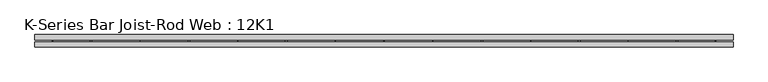
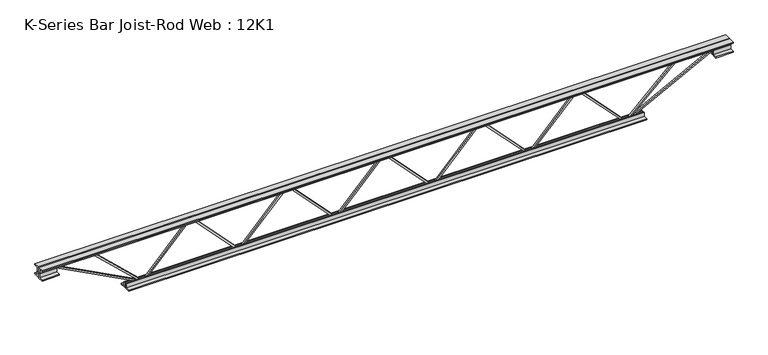
"""IFC4 building model written with IfcOpenShell, lengths in millimetres: beam geometry, K-Series Bar Joist-Rod Web : 12K1."""

from ifc_helpers import new_model, si_unit, frame, origin, place, context, project, spatial, polyline, outline, extrude, source, transform, mapped, element, save


def k_series_bar_joist_rod_web_12k1_58f41b11(model_context):
    return source(origin(), model_context, "Body", "SweptSolid", [
        extrude(outline(polyline([(-141.2875, 283.68625), (-150.8125, 283.68625), (-150.8125, 288.9066515), (141.2875, 566.2429015), (141.2875, 568.5020985), (-150.8125, 845.8383485), (-150.8125, 851.05875), (-141.2875, 851.05875), (-141.2875, 849.9291515), (150.8125, 572.5929015), (150.8125, 562.1520985), (-141.2875, 284.8158485), (-141.2875, 283.68625)])), frame((0.0, -4.7625, 0.0), z_axis=(0.0, 1.0, 0.0), x_axis=(0.0, 0.0, 1.0)), (0.0, 0.0, 1.0), 9.525),
        extrude(outline(polyline([(-141.2875, -283.68625), (-150.8125, -283.68625), (-150.8125, -278.4658485), (141.2875, -1.1295985), (141.2875, 1.1295985), (-150.8125, 278.4658485), (-150.8125, 283.68625), (-141.2875, 283.68625), (-141.2875, 282.5566515), (150.8125, 5.2204015), (150.8125, -5.2204015), (-141.2875, -282.5566515), (-141.2875, -283.68625)])), frame((0.0, -4.7625, 0.0), z_axis=(0.0, 1.0, 0.0), x_axis=(0.0, 0.0, 1.0)), (0.0, 0.0, 1.0), 9.525),
        extrude(outline(polyline([(-141.2875, -851.05875), (-150.8125, -851.05875), (-150.8125, -845.8383485), (141.2875, -568.5020985), (141.2875, -566.2429015), (-150.8125, -288.9066515), (-150.8125, -283.68625), (-141.2875, -283.68625), (-141.2875, -284.8158485), (150.8125, -562.1520985), (150.8125, -572.5929015), (-141.2875, -849.9291515), (-141.2875, -851.05875)])), frame((0.0, -4.7625, 0.0), z_axis=(0.0, 1.0, 0.0), x_axis=(0.0, 0.0, 1.0)), (0.0, 0.0, 1.0), 9.525),
        extrude(outline(polyline([(-141.2875, 851.05875), (-150.8125, 851.05875), (-150.8125, 856.2791515), (141.2875, 1133.6154015), (141.2875, 1135.8745985), (-150.8125, 1413.2108485), (-150.8125, 1418.43125), (-141.2875, 1418.43125), (-141.2875, 1417.3016515), (150.8125, 1139.9654015), (150.8125, 1129.5245985), (-141.2875, 852.1883485), (-141.2875, 851.05875)])), frame((0.0, -4.7625, 0.0), z_axis=(0.0, 1.0, 0.0), x_axis=(0.0, 0.0, 1.0)), (0.0, 0.0, 1.0), 9.525),
        extrude(outline(polyline([(-141.2875, -1418.43125), (-150.8125, -1418.43125), (-150.8125, -1413.2108485), (141.2875, -1135.8745985), (141.2875, -1133.6154015), (-150.8125, -856.2791515), (-150.8125, -851.05875), (-141.2875, -851.05875), (-141.2875, -852.1883485), (150.8125, -1129.5245985), (150.8125, -1139.9654015), (-141.2875, -1417.3016515), (-141.2875, -1418.43125)])), frame((0.0, -4.7625, 0.0), z_axis=(0.0, 1.0, 0.0), x_axis=(0.0, 0.0, 1.0)), (0.0, 0.0, 1.0), 9.525),
        extrude(outline(polyline([(4.7625, 152.4), (36.5125, 152.4), (36.5125, 146.05), (11.1125, 146.05), (11.1125, 120.65), (4.7625, 120.65), (4.7625, 152.4)])), frame((-2028.03125, 0.0, 0.0), z_axis=(1.0, 0.0, 0.0), x_axis=(0.0, 1.0, 0.0)), (0.0, 0.0, 1.0), 4056.0625),
        extrude(outline(polyline([(-4.7625, 152.4), (-4.7625, 120.65), (-11.1125, 120.65), (-11.1125, 146.05), (-36.5125, 146.05), (-36.5125, 152.4), (-4.7625, 152.4)])), frame((-2028.03125, 0.0, 0.0), z_axis=(1.0, 0.0, 0.0), x_axis=(0.0, 1.0, 0.0)), (0.0, 0.0, 1.0), 4056.0625),
        extrude(outline(polyline([(-4.7625, 88.9), (-36.5125, 88.9), (-36.5125, 95.25), (-11.1125, 95.25), (-11.1125, 120.65), (-4.7625, 120.65), (-4.7625, 88.9)])), frame((-2028.03125, 0.0, 0.0), z_axis=(1.0, 0.0, 0.0), x_axis=(0.0, 1.0, 0.0)), (0.0, 0.0, 1.0), 101.6),
        extrude(outline(polyline([(36.5125, 88.9), (4.7625, 88.9), (4.7625, 120.65), (11.1125, 120.65), (11.1125, 95.25), (36.5125, 95.25), (36.5125, 88.9)])), frame((-2028.03125, 0.0, 0.0), z_axis=(1.0, 0.0, 0.0), x_axis=(0.0, 1.0, 0.0)), (0.0, 0.0, 1.0), 101.6),
        extrude(outline(polyline([(4.7625, 88.9), (4.7625, 120.65), (11.1125, 120.65), (11.1125, 95.25), (36.5125, 95.25), (36.5125, 88.9), (4.7625, 88.9)])), frame((1926.43125, 0.0, 0.0), z_axis=(1.0, 0.0, 0.0), x_axis=(0.0, 1.0, 0.0)), (0.0, 0.0, 1.0), 101.6),
        extrude(outline(polyline([(-4.7625, 88.9), (-36.5125, 88.9), (-36.5125, 95.25), (-11.1125, 95.25), (-11.1125, 120.65), (-4.7625, 120.65), (-4.7625, 88.9)])), frame((1926.43125, 0.0, 0.0), z_axis=(1.0, 0.0, 0.0), x_axis=(0.0, 1.0, 0.0)), (0.0, 0.0, 1.0), 101.6),
        extrude(outline(polyline([(4.7625, -152.4), (4.7625, -120.65), (11.1125, -120.65), (11.1125, -146.05), (36.5125, -146.05), (36.5125, -152.4), (4.7625, -152.4)])), frame((-1520.03125, 0.0, 0.0), z_axis=(1.0, 0.0, 0.0), x_axis=(0.0, 1.0, 0.0)), (0.0, 0.0, 1.0), 3040.0625),
        extrude(outline(polyline([(-4.7625, -152.4), (-36.5125, -152.4), (-36.5125, -146.05), (-11.1125, -146.05), (-11.1125, -120.65), (-4.7625, -120.65), (-4.7625, -152.4)])), frame((-1520.03125, 0.0, 0.0), z_axis=(1.0, 0.0, 0.0), x_axis=(0.0, 1.0, 0.0)), (0.0, 0.0, 1.0), 3040.0625),
        extrude(outline(polyline([(0.0, -9.525), (0.0, 0.0), (573.7533355, 0.0), (573.7533355, -9.525), (0.0, -9.525)])), frame((-1928.6450214, 4.7625, 116.4332925), z_axis=(0.4648338989895146, 0.0, 0.8853979028381566), x_axis=(0.8853979028381566, 0.0, -0.4648338989895146)), (0.0, 0.0, 1.0), 9.525),
        extrude(outline(polyline([(0.0, -9.525), (0.0, 0.0), (389.3671512, 0.0), (389.3671512, -9.525), (0.0, -9.525)])), frame((-1705.3796107, 4.7625, 117.1801239), z_axis=(0.6849576271986557, 0.0, 0.7285829046459898), x_axis=(0.7285829046459898, 0.0, -0.6849576271986557)), (0.0, 0.0, 1.0), 9.525),
        extrude(outline(polyline([(0.0, -9.525), (0.0, 0.0), (573.7533355, 0.0), (573.7533355, -9.525), (0.0, -9.525)])), frame((1928.6450214, -4.7625, 116.4332925), z_axis=(-0.4648338989894953, 0.0, 0.8853979028381667), x_axis=(-0.8853979028381667, 0.0, -0.4648338989894953)), (0.0, 0.0, 1.0), 9.525),
        extrude(outline(polyline([(0.0, -9.525), (0.0, 0.0), (389.3671512, 0.0), (389.3671512, -9.525), (0.0, -9.525)])), frame((1705.3796107, -4.7625, 117.1801239), z_axis=(-0.6849576271986486, 0.0, 0.7285829046459964), x_axis=(-0.7285829046459964, 0.0, -0.6849576271986486)), (0.0, 0.0, 1.0), 9.525),
    ])


if __name__ == "__main__":
    model = new_model("IFC4")
    model_context = context("Model", 3, world=origin())
    ifc_project = project(units=[si_unit("LENGTHUNIT", "METRE", prefix="MILLI")], contexts=[model_context])
    site = spatial("IfcSite", under=ifc_project)
    building = spatial("IfcBuilding", under=site)
    placement = place(None, origin())
    k_series_bar_joist_rod_web_12k1_shape = k_series_bar_joist_rod_web_12k1_58f41b11(model_context)
    element("IfcBeam", 1, ObjectType="K-Series Bar Joist-Rod Web : 12K1", at=placement, inside=building, context=model_context, shape_type="MappedRepresentation", body=[
        mapped(k_series_bar_joist_rod_web_12k1_shape, transform((0.0, 0.0, 0.0), x_axis=(1.0, 0.0, 0.0), y_axis=(0.0, 1.0, 0.0), z_axis=(0.0, 0.0, 1.0))),
    ])
    save(model, "model.ifc")

# Revit data of these elements
# Type "K-Series Bar Joist-Rod Web : 12K1"
#   Assembly Code = "B1010350"
#   Wt = 5
#   Web Thickness = 0' - 0 3/8"
#   Start Offset [instance default] = 0' - 0"
#   Start Extension [instance default] = 0' - 0"
#   Seat Length = 0' - 4"
#   Seat Depth = 0' - 2 1/2"
#   PanelArrayLength [instance default] = 20' - 0"
#   Panel [instance default] = 2' - 0"
#   End Offset [instance default] = 0' - 0"
#   End Extension [instance default] = 0' - 0"
#   End Panel = 2' - 0"
#   Cord Leg = 0' - 1 1/4"
#   Chord Thickness = 0' - 0 1/4"
#   Length [instance default] = 24' - 0"
#   Depth = 1' - 0"
#   PanelArrayNum [instance default] = 10
#   Structural Material = none
# Element 1 (IfcBeam, "K-Series Bar Joist-Rod Web : 12K1")
#   PanelArrayLength = 9' - 3 11/16"
#   Panel = 1' - 10.3375"
#   PanelArrayNum = 5
